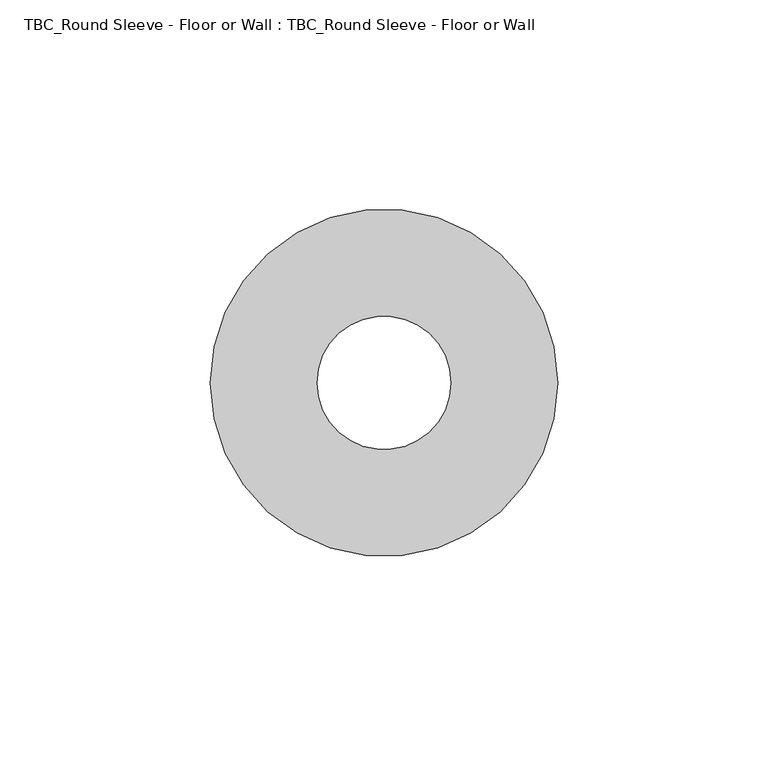
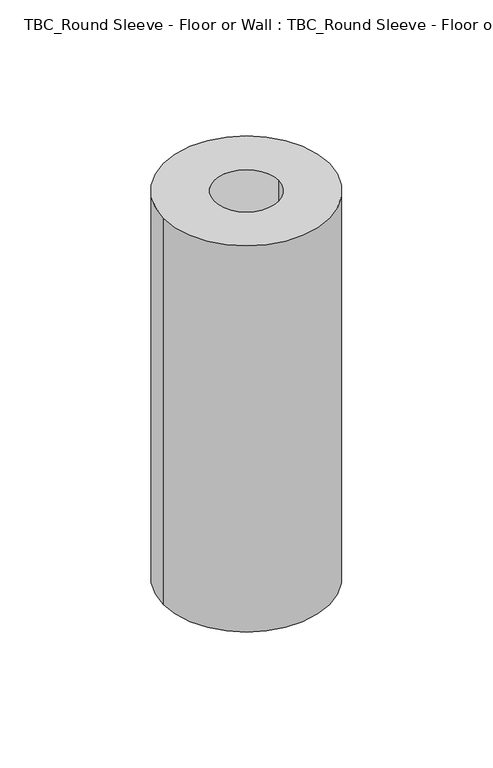
"""IFC4 building model written with IfcOpenShell, lengths in millimetres: proxy geometry, TBC_Round Sleeve - Floor or Wall : TBC_Round Sleeve - Floor or Wall."""

from ifc_helpers import new_model, si_unit, point, frame, origin, origin_2d, place, context, project, spatial, circle_curve, trimmed, segment, composite_curve, outline, extrude, source, transform, mapped, element, save


def tbc_round_sleeve_floor_or_wall_tbc_round_sleeve_floor_or_d2dd5259(model_context):
    return source(origin(), model_context, "Body", "SweptSolid", [
        extrude(outline(composite_curve([segment(trimmed(circle_curve(origin_2d(), 41.275), [point((-41.275, 0.0))], [point((41.275, 0.0))], False, "CARTESIAN"), True, "CONTINUOUS"), segment(trimmed(circle_curve(origin_2d(), 41.275), [point((41.275, 0.0))], [point((-41.275, 0.0))], False, "CARTESIAN"), True, "CONTINUOUS")], self_intersect=False), holes=[composite_curve([segment(trimmed(circle_curve(origin_2d(), 15.875), [point((-15.875, 0.0))], [point((15.875, 0.0))], True, "CARTESIAN"), True, "CONTINUOUS"), segment(trimmed(circle_curve(origin_2d(), 15.875), [point((15.875, 0.0))], [point((-15.875, 0.0))], True, "CARTESIAN"), True, "CONTINUOUS")], self_intersect=False)]), frame((0.0, 0.0, -203.2), z_axis=(0.0, 0.0, 1.0), x_axis=(1.0, 0.0, 0.0)), (0.0, 0.0, 1.0), 203.2),
    ])


if __name__ == "__main__":
    model = new_model("IFC4")
    model_context = context("Model", 3, world=origin())
    ifc_project = project(units=[si_unit("LENGTHUNIT", "METRE", prefix="MILLI")], contexts=[model_context])
    site = spatial("IfcSite", under=ifc_project)
    building = spatial("IfcBuilding", under=site)
    placement = place(None, origin())
    tbc_round_sleeve_floor_or_wall_tbc_round_sleeve_floor_or_shape = tbc_round_sleeve_floor_or_wall_tbc_round_sleeve_floor_or_d2dd5259(model_context)
    element("IfcBuildingElementProxy", 1, Name="TBC_Round Sleeve - Floor or Wall : TBC_Round Sleeve - Floor or Wall", ObjectType="TBC_Round Sleeve - Floor or Wall : TBC_Round Sleeve - Floor or Wall", at=placement, inside=building, context=model_context, shape_type="MappedRepresentation", body=[
        mapped(tbc_round_sleeve_floor_or_wall_tbc_round_sleeve_floor_or_shape, transform((0.0, 0.0, 0.0), x_axis=(1.0, 0.0, 0.0), y_axis=(0.0, 1.0, 0.0), z_axis=(0.0, 0.0, 1.0))),
    ])
    save(model, "model.ifc")

# Revit data of these elements
# Type "TBC_Round Sleeve - Floor or Wall : TBC_Round Sleeve - Floor or Wall"
#   Tag Dimension [instance default] = ""
#   MEP Type [instance default] = ""
#   MEP Element [instance default] = ""
#   MEP Category [instance default] = ""
#   Host Element Type [instance default] = ""
#   Host Element Id [instance default] = ""
#   Host Element Category [instance default] = ""
#   Control Line Y [instance default] = ""
#   Control Line X [instance default] = ""
#   Sleeve Radius [instance default] = 1' - 0"
#   Sleeve Edge [instance default] = 1' - 2"
#   Sleeve Depth [instance default] = 3' - 0"
#   Distance Y [instance default] = 0' - 0"
#   Distance X [instance default] = 0' - 0"
#   Default Elevation = 0
# Element 1 (IfcBuildingElementProxy, "TBC_Round Sleeve - Floor or Wall : TBC_Round Sleeve - Floor or Wall")
#   Tag Dimension = "1.25\"ø"
#   MEP Type = "Mechanical-CWR"
#   MEP Element = "562707"
#   MEP Category = "Pipe"
#   Host Element Type = "8\" Plank"
#   Host Element Id = "732720"
#   Host Element Category = "Floors"
#   Sleeve Radius = 0' - 1 1/4"
#   Sleeve Edge = 0' - 3 1/4"
#   Sleeve Depth = 0' - 8"
